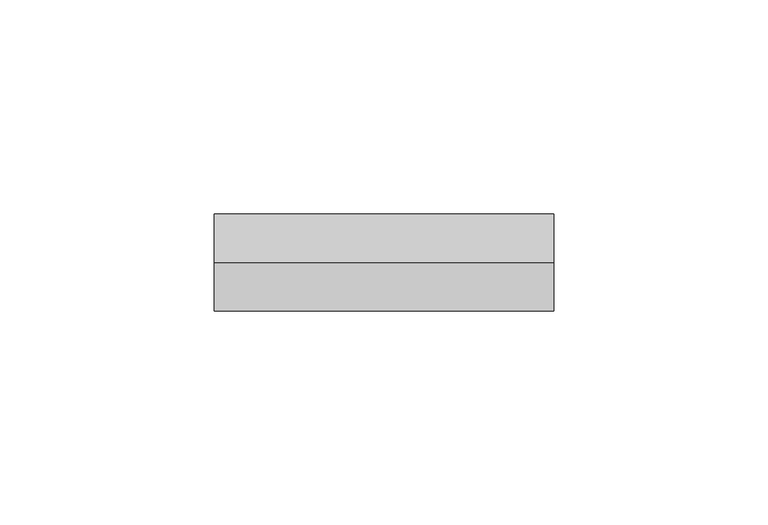
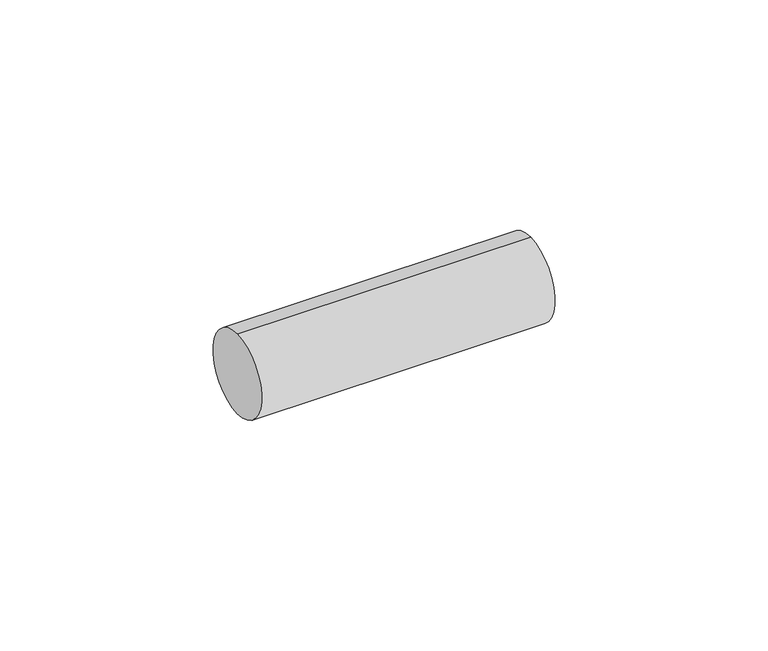
"""IFC4 building model written with IfcOpenShell, lengths in millimetres: proxy geometry, Bolt28:Bolt003:304731 : Bolt28:Bolt003:304731."""

from ifc_helpers import new_model, si_unit, point, frame, frame_2d, origin, place, context, project, spatial, circle_curve, trimmed, segment, composite_curve, outline, extrude, source, transform, mapped, element, save


def generic_models_a3ebc139(model_context):
    return source(origin(), model_context, "Body", "SweptSolid", [
        extrude(outline(composite_curve([segment(trimmed(circle_curve(frame_2d((2264.1630212, 40070.0545241)), 11.4045168), [point((2264.1630212, 40058.6500073))], [point((2264.1630212, 40081.4590409))], False, "CARTESIAN"), True, "CONTINUOUS"), segment(trimmed(circle_curve(frame_2d((2264.1630212, 40070.0545241)), 11.4045168), [point((2264.1630212, 40081.4590409))], [point((2264.1630212, 40058.6500073))], False, "CARTESIAN"), True, "CONTINUOUS")], self_intersect=False)), frame((15042.0981889, 0.0, 0.0), z_axis=(1.0, 0.0, 0.0), x_axis=(0.0, 1.0, 0.0)), (0.0, 0.0, 1.0), 79.375),
    ])


if __name__ == "__main__":
    model = new_model("IFC4")
    model_context = context("Model", 3, world=origin())
    ifc_project = project(units=[si_unit("LENGTHUNIT", "METRE", prefix="MILLI")], contexts=[model_context])
    site = spatial("IfcSite", under=ifc_project)
    building = spatial("IfcBuilding", under=site)
    placement = place(None, origin())
    generic_models_shape = generic_models_a3ebc139(model_context)
    element("IfcBuildingElementProxy", 1, Name="Bolt28:Bolt003:304731 : Bolt28:Bolt003:304731", ObjectType="Bolt28:Bolt003:304731 : Bolt28:Bolt003:304731", at=placement, inside=building, context=model_context, shape_type="MappedRepresentation", body=[
        mapped(generic_models_shape, transform((0.0, 0.0, 0.0), x_axis=(1.0, 0.0, 0.0), y_axis=(0.0, 1.0, 0.0), z_axis=(0.0, 0.0, 1.0))),
    ])
    save(model, "model.ifc")

# Revit data of these elements
# Type "Bolt28:Bolt003:304731 : Bolt28:Bolt003:304731"
#   NameOverride = "Bolt28:Bolt003:304731"
#   ObjectTypeOverride = "Bolt28:Bolt003"
#   Reference = "Bolt003"
#   Category = "Generic Models"
#   Tag = "304731"
# Element 1 (IfcBuildingElementProxy, "Bolt28:Bolt003:304731 : Bolt28:Bolt003:304731")
#   Materials on its faces: "TUBE STEEL STRINGER WELDED TO ANCHORED STEEL PLATE - SEE STRUCT DWGS"
# Materials
#   "TUBE STEEL STRINGER WELDED TO ANCHORED STEEL PLATE - SEE STRUCT DWGS": class "Unassigned", colour RGB 128 128 128, transparency 0, Cost = 0
